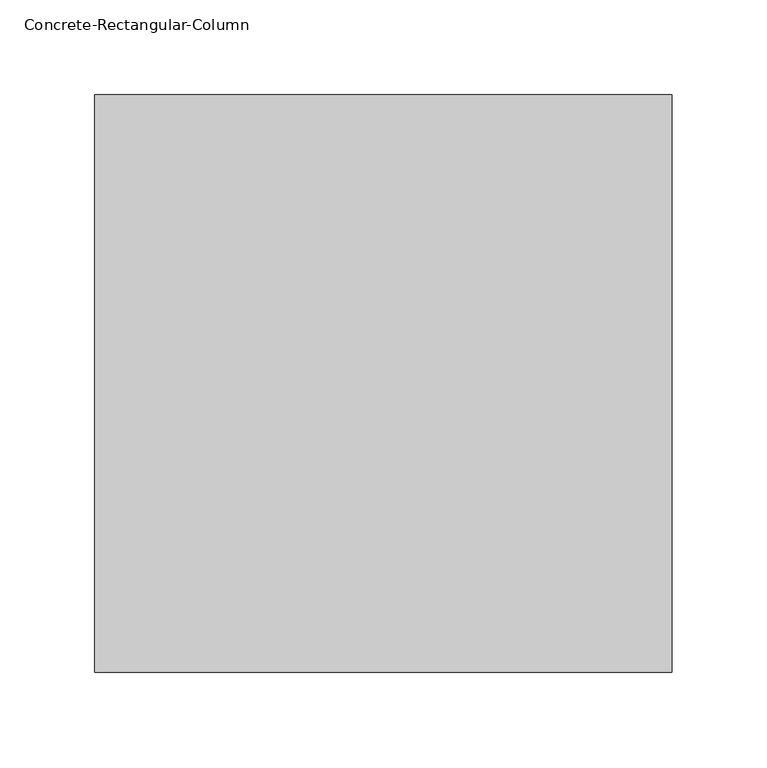
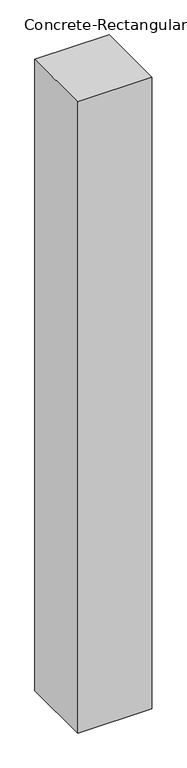
"""IFC4 building model written with IfcOpenShell, lengths in millimetres: column geometry, Concrete-Rectangular-Column : 12*12 Column."""

import ifcopenshell
import ifcopenshell.guid

model = None  # the IFC model being written
_history = None  # IfcOwnerHistory: only IFC2X3 demands one
_inside = {}  # id of a spatial element -> (the spatial element, [elements in it])
_under = {}  # id of a project, library or spatial element -> (it, [spatial elements below it])
_declared = {}  # id of a project -> (the project, [libraries it declares])
_typed = {}  # id of a type object -> (the type object, [elements of that type])
_made_of = {}  # id of a material, layer set ... -> (it, [elements and type objects made of it])


def new_model(schema):
    """Start an empty IFC model of exactly this schema.

    Asked for "IFC4X3", IfcOpenShell would pick the latest addendum, in which some entities
    have other attributes; the version numbers below select the first issue.
    IFC2X3 requires an IfcOwnerHistory on every rooted entity: one is made here for all.
    """
    global model, _history
    if schema == "IFC4X3":
        model = ifcopenshell.file(schema_version=(4, 3, 0, 0))
    else:
        model = ifcopenshell.file(schema=schema)
    _inside.clear()
    _under.clear()
    _declared.clear()
    _typed.clear()
    _made_of.clear()
    _history = None
    if model.schema == "IFC2X3":
        org = make("IfcOrganization", Name="unknown")
        user = make(
            "IfcPersonAndOrganization",
            ThePerson=make("IfcPerson", FamilyName="unknown"),
            TheOrganization=org,
        )
        app = make(
            "IfcApplication",
            ApplicationDeveloper=org,
            Version="unknown",
            ApplicationFullName="unknown",
            ApplicationIdentifier="unknown",
        )
        _history = make(
            "IfcOwnerHistory",
            OwningUser=user,
            OwningApplication=app,
            ChangeAction="ADDED",
            CreationDate=0,
        )
    return model


def make(cls, **values):
    """One entity of the class cls with the attributes given. An attribute that is None is left unset."""
    return model.create_entity(
        cls, **{name: value for name, value in values.items() if value is not None}
    )


def rooted(cls, **values):
    """An entity with a GlobalId (a new one), such as an element, a storey or a relation."""
    return make(cls, GlobalId=ifcopenshell.guid.new(), OwnerHistory=_history, **values)


def si_unit(unit_type, name, prefix=None):
    """IfcSIUnit, for example si_unit("LENGTHUNIT", "METRE", prefix="MILLI")."""
    return make("IfcSIUnit", UnitType=unit_type, Prefix=prefix, Name=name)


def assignment(units):
    """IfcUnitAssignment: the units of a project."""
    return None if units is None else make("IfcUnitAssignment", Units=units)


def point(xyz):
    """IfcCartesianPoint."""
    return None if xyz is None else make("IfcCartesianPoint", Coordinates=xyz)


def direction(xyz):
    """IfcDirection."""
    return None if xyz is None else make("IfcDirection", DirectionRatios=xyz)


def frame(location, z_axis=None, x_axis=None):
    """IfcAxis2Placement3D, a coordinate frame: its origin and axes. An axis left out is left unset."""
    return make(
        "IfcAxis2Placement3D",
        Location=point(location),
        Axis=direction(z_axis),
        RefDirection=direction(x_axis),
    )


def origin():
    """The frame at (0, 0, 0) with its axes left unset."""
    return frame((0.0, 0.0, 0.0))


def place(relative_to, where):
    """IfcLocalPlacement: puts the frame where relative to a parent placement (None: the world)."""
    return make(
        "IfcLocalPlacement", PlacementRelTo=relative_to, RelativePlacement=where
    )


def context(
    kind, dimensions, precision=None, world=None, true_north=None, identifier=None
):
    """IfcGeometricRepresentationContext, for example the 3D "Model" context."""
    return make(
        "IfcGeometricRepresentationContext",
        ContextIdentifier=identifier,
        ContextType=kind,
        CoordinateSpaceDimension=dimensions,
        Precision=precision,
        WorldCoordinateSystem=world,
        TrueNorth=true_north,
    )


def project(units=None, contexts=None):
    """IfcProject with its units and contexts."""
    return rooted(
        "IfcProject",
        Name="project",
        RepresentationContexts=contexts,
        UnitsInContext=assignment(units),
    )


def spatial(cls, under=None, at=None, **own):
    """A site, building, storey or space (cls), placed at a placement, below another one or the project."""
    s = rooted(cls, ObjectPlacement=at, **own)
    if under is not None:
        _under.setdefault(under.id(), (under, []))[1].append(s)
    return s


def polyline(points):
    """IfcPolyline through the points."""
    return make("IfcPolyline", Points=[point(p) for p in points])


def outline(outer, holes=None, kind="AREA"):
    """IfcArbitraryClosedProfileDef: a profile drawn as a closed curve; with holes, ...WithVoids."""
    if holes is None:
        return make("IfcArbitraryClosedProfileDef", ProfileType=kind, OuterCurve=outer)
    return make(
        "IfcArbitraryProfileDefWithVoids",
        ProfileType=kind,
        OuterCurve=outer,
        InnerCurves=holes,
    )


def extrude(swept, where, along, depth):
    """IfcExtrudedAreaSolid: the profile swept, set in the frame where, extruded along a direction by depth."""
    return make(
        "IfcExtrudedAreaSolid",
        SweptArea=swept,
        Position=where,
        ExtrudedDirection=direction(along),
        Depth=depth,
    )


def shape(context_of_items, identifier, shape_type, items):
    """IfcShapeRepresentation: the items that make up one representation, for example the "Body"."""
    return make(
        "IfcShapeRepresentation",
        ContextOfItems=context_of_items,
        RepresentationIdentifier=identifier,
        RepresentationType=shape_type,
        Items=items,
    )


def source(mapping_origin, context_of_items, identifier, shape_type, items):
    """IfcRepresentationMap: a shape defined once, which mapped items show again and again."""
    return make(
        "IfcRepresentationMap",
        MappingOrigin=mapping_origin,
        MappedRepresentation=shape(context_of_items, identifier, shape_type, items),
    )


def transform(
    local_origin,
    x_axis=None,
    y_axis=None,
    z_axis=None,
    scale=None,
    scale2=None,
    scale3=None,
    uniform=True,
):
    """IfcCartesianTransformationOperator3D, or its non-uniform kind. x_axis, y_axis, z_axis: its Axis1, 2, 3."""
    if uniform:
        return make(
            "IfcCartesianTransformationOperator3D",
            Axis1=direction(x_axis),
            Axis2=direction(y_axis),
            LocalOrigin=point(local_origin),
            Scale=scale,
            Axis3=direction(z_axis),
        )
    return make(
        "IfcCartesianTransformationOperator3DnonUniform",
        Axis1=direction(x_axis),
        Axis2=direction(y_axis),
        LocalOrigin=point(local_origin),
        Scale=scale,
        Axis3=direction(z_axis),
        Scale2=scale2,
        Scale3=scale3,
    )


def mapped(mapping_source, mapping_target):
    """IfcMappedItem: shows the shape of a source again, moved by a transform."""
    return make(
        "IfcMappedItem", MappingSource=mapping_source, MappingTarget=mapping_target
    )


def made_of(thing, what):
    """Note that an element or type object is made of a material, layer set ...; save() writes the relation."""
    if what is not None:
        _made_of.setdefault(what.id(), (what, []))[1].append(thing)
    return thing


def element(
    cls,
    number,
    at=None,
    inside=None,
    cuts=None,
    type_object=None,
    material=None,
    context=None,
    identifier="Body",
    shape_type=None,
    held_by="IfcProductDefinitionShape",
    body=None,
    shapes=None,
    **own,
):
    """One element of the class cls, such as IfcWall. Its Tag is "e" and its number.

    at: its placement. inside: the storey or other place that contains it. cuts: it is an
    opening in that element (IfcRelVoidsElement). A single representation is given by context,
    identifier, shape_type and body (its items); several are given by shapes. held_by: the class
    of the entity that holds the representations. save() writes the other relations.
    """
    e = rooted(cls, Tag="e%d" % number, ObjectPlacement=at, **own)
    if body is not None:
        shapes = [shape(context, identifier, shape_type, body)]
    if shapes is not None:
        e.Representation = make(held_by, Representations=shapes)
    if inside is not None:
        _inside.setdefault(inside.id(), (inside, []))[1].append(e)
    if cuts is not None:
        rooted(
            "IfcRelVoidsElement", RelatingBuildingElement=cuts, RelatedOpeningElement=e
        )
    if type_object is not None:
        _typed.setdefault(type_object.id(), (type_object, []))[1].append(e)
    return made_of(e, material)


def aggregate(whole, parts):
    """IfcRelAggregates: a whole, such as a stair, and the parts it consists of."""
    return rooted("IfcRelAggregates", RelatingObject=whole, RelatedObjects=parts)


def save(model, path):
    """Write the relations noted so far, then the file.

    IfcRelAggregates (storeys below a building ...), IfcRelContainedInSpatialStructure (elements
    in a storey), IfcRelDefinesByType, IfcRelAssociatesMaterial and IfcRelDeclares: one each for
    every whole, place, type object, material and project.
    """
    for whole, parts in _under.values():
        aggregate(whole, parts)
    for where, things in _inside.values():
        rooted(
            "IfcRelContainedInSpatialStructure",
            RelatedElements=things,
            RelatingStructure=where,
        )
    for kind, things in _typed.values():
        rooted("IfcRelDefinesByType", RelatedObjects=things, RelatingType=kind)
    for what, things in _made_of.values():
        rooted("IfcRelAssociatesMaterial", RelatedObjects=things, RelatingMaterial=what)
    for by, libraries in _declared.values():
        rooted("IfcRelDeclares", RelatingContext=by, RelatedDefinitions=libraries)
    model.write(path)


def concrete_rectangular_column_483f9928(model_context):
    return source(origin(), model_context, "Body", "SweptSolid", [
        extrude(outline(polyline([(152.4, 152.4), (152.4, -152.4), (-152.4, -152.4), (-152.4, 152.4), (152.4, 152.4)])), frame((0.0, 0.0, 5740.4), z_axis=(0.0, 0.0, 1.0), x_axis=(1.0, 0.0, 0.0)), (0.0, 0.0, 1.0), 2743.2),
    ])


if __name__ == "__main__":
    model = new_model("IFC4")
    model_context = context("Model", 3, world=origin())
    ifc_project = project(units=[si_unit("LENGTHUNIT", "METRE", prefix="MILLI")], contexts=[model_context])
    site = spatial("IfcSite", under=ifc_project)
    building = spatial("IfcBuilding", under=site)
    placement = place(None, origin())
    concrete_rectangular_column_shape = concrete_rectangular_column_483f9928(model_context)
    element("IfcColumn", 1, ObjectType="Concrete-Rectangular-Column : 12*12 Column", at=placement, inside=building, context=model_context, shape_type="MappedRepresentation", body=[
        mapped(concrete_rectangular_column_shape, transform((0.0, 0.0, 0.0), x_axis=(1.0, 0.0, 0.0), y_axis=(0.0, 1.0, 0.0), z_axis=(0.0, 0.0, 1.0))),
    ])
    save(model, "model.ifc")

# Revit data of these elements
# Project information
#   Project Issue Date = "Issue Date"
#   Project Status = "Project Status"
#   Client Name = "Owner"
#   Project Address = "Enter address here"
#   Project Name = "Project Name"
#   Project Number = "Project Number"
# Type "Concrete-Rectangular-Column : 12*12 Column"
#   Assembly Code = "B10"
#   b = 1' - 0"
#   h = 1' - 0"
#   Structural Material [instance default] = Concrete, Cast-in-Place gray
# Element 1 (IfcColumn, "Concrete-Rectangular-Column : 12*12 Column")
#   Materials on its faces: "Concrete, Cast-in-Place gray"
# Materials
#   "Concrete, Cast-in-Place gray": class "Concrete", colour RGB 192 192 192, transparency 0, Description = "Cast-in-place concrete", Cost = 0
